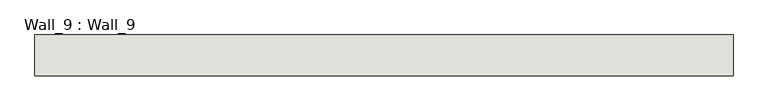
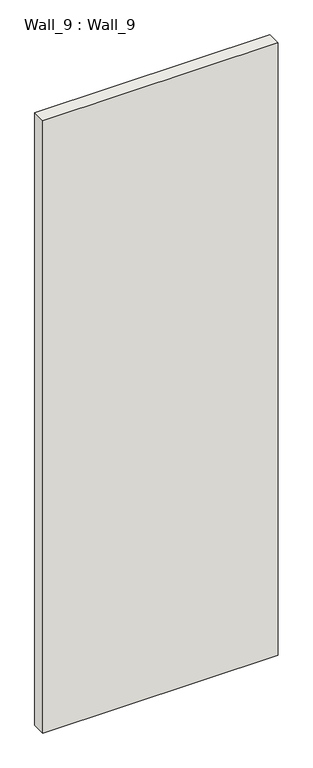
"""IFC4 building model written with IfcOpenShell, lengths in millimetres: wall geometry, Wall_9 : Wall_9."""

from ifc_helpers import new_model, si_unit, origin, origin_with_axes, place, context, project, spatial, polyline, outline, extrude, source, transform, mapped, element, save


def wall_9_wall_9_7e9080d3(model_context):
    return source(origin(), model_context, "Body", "SweptSolid", [
        extrude(outline(polyline([(6190.0, 11990.0), (4480.0, 11990.0), (4480.0, 12090.0), (6190.0, 12090.0), (6190.0, 11990.0)])), origin_with_axes(), (0.0, 0.0, 1.0), 4700.0),
    ])


if __name__ == "__main__":
    model = new_model("IFC4")
    model_context = context("Model", 3, world=origin())
    ifc_project = project(units=[si_unit("LENGTHUNIT", "METRE", prefix="MILLI")], contexts=[model_context])
    site = spatial("IfcSite", under=ifc_project)
    building = spatial("IfcBuilding", under=site)
    placement = place(None, origin())
    wall_9_wall_9_shape = wall_9_wall_9_7e9080d3(model_context)
    element("IfcWall", 1, ObjectType="Wall_9 : Wall_9", at=placement, inside=building, context=model_context, shape_type="MappedRepresentation", body=[
        mapped(wall_9_wall_9_shape, transform((0.0, 0.0, 0.0), x_axis=(1.0, 0.0, 0.0), y_axis=(0.0, 1.0, 0.0), z_axis=(0.0, 0.0, 1.0))),
    ])
    save(model, "model.ifc")

# Revit data of these elements
# Type "Wall_9 : Wall_9"
#   NameOverride = "Wall_9"
# Element 1 (IfcWall, "Wall_9 : Wall_9")
#   Materials on its faces: "IfcSurfaceStyle #33"
# Materials
#   "IfcSurfaceStyle #33": class "Unassigned", colour RGB 214 214 214, transparency 0
